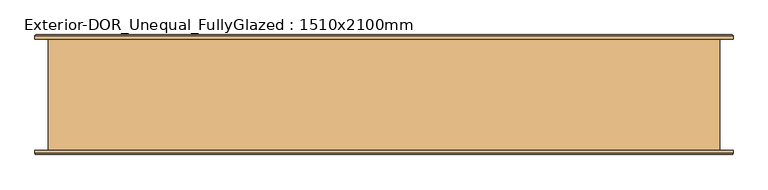
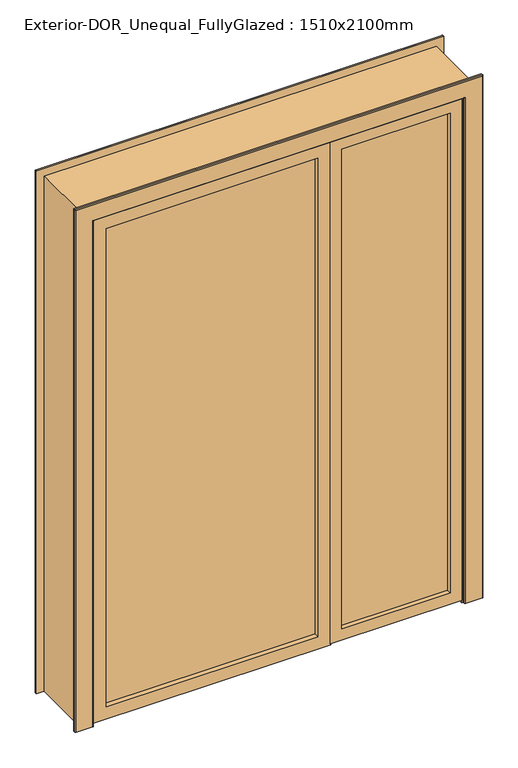
"""IFC4 building model written with IfcOpenShell, lengths in millimetres: door geometry, Exterior-DOR_Unequal_FullyGlazed : 1510x2100mm."""

import ifcopenshell
import ifcopenshell.guid

model = None  # the IFC model being written
_history = None  # IfcOwnerHistory: only IFC2X3 demands one
_inside = {}  # id of a spatial element -> (the spatial element, [elements in it])
_under = {}  # id of a project, library or spatial element -> (it, [spatial elements below it])
_declared = {}  # id of a project -> (the project, [libraries it declares])
_typed = {}  # id of a type object -> (the type object, [elements of that type])
_made_of = {}  # id of a material, layer set ... -> (it, [elements and type objects made of it])


def new_model(schema):
    """Start an empty IFC model of exactly this schema.

    Asked for "IFC4X3", IfcOpenShell would pick the latest addendum, in which some entities
    have other attributes; the version numbers below select the first issue.
    IFC2X3 requires an IfcOwnerHistory on every rooted entity: one is made here for all.
    """
    global model, _history
    if schema == "IFC4X3":
        model = ifcopenshell.file(schema_version=(4, 3, 0, 0))
    else:
        model = ifcopenshell.file(schema=schema)
    _inside.clear()
    _under.clear()
    _declared.clear()
    _typed.clear()
    _made_of.clear()
    _history = None
    if model.schema == "IFC2X3":
        org = make("IfcOrganization", Name="unknown")
        user = make(
            "IfcPersonAndOrganization",
            ThePerson=make("IfcPerson", FamilyName="unknown"),
            TheOrganization=org,
        )
        app = make(
            "IfcApplication",
            ApplicationDeveloper=org,
            Version="unknown",
            ApplicationFullName="unknown",
            ApplicationIdentifier="unknown",
        )
        _history = make(
            "IfcOwnerHistory",
            OwningUser=user,
            OwningApplication=app,
            ChangeAction="ADDED",
            CreationDate=0,
        )
    return model


def make(cls, **values):
    """One entity of the class cls with the attributes given. An attribute that is None is left unset."""
    return model.create_entity(
        cls, **{name: value for name, value in values.items() if value is not None}
    )


def rooted(cls, **values):
    """An entity with a GlobalId (a new one), such as an element, a storey or a relation."""
    return make(cls, GlobalId=ifcopenshell.guid.new(), OwnerHistory=_history, **values)


def si_unit(unit_type, name, prefix=None):
    """IfcSIUnit, for example si_unit("LENGTHUNIT", "METRE", prefix="MILLI")."""
    return make("IfcSIUnit", UnitType=unit_type, Prefix=prefix, Name=name)


def assignment(units):
    """IfcUnitAssignment: the units of a project."""
    return None if units is None else make("IfcUnitAssignment", Units=units)


def point(xyz):
    """IfcCartesianPoint."""
    return None if xyz is None else make("IfcCartesianPoint", Coordinates=xyz)


def direction(xyz):
    """IfcDirection."""
    return None if xyz is None else make("IfcDirection", DirectionRatios=xyz)


def frame(location, z_axis=None, x_axis=None):
    """IfcAxis2Placement3D, a coordinate frame: its origin and axes. An axis left out is left unset."""
    return make(
        "IfcAxis2Placement3D",
        Location=point(location),
        Axis=direction(z_axis),
        RefDirection=direction(x_axis),
    )


def origin():
    """The frame at (0, 0, 0) with its axes left unset."""
    return frame((0.0, 0.0, 0.0))


def place(relative_to, where):
    """IfcLocalPlacement: puts the frame where relative to a parent placement (None: the world)."""
    return make(
        "IfcLocalPlacement", PlacementRelTo=relative_to, RelativePlacement=where
    )


def context(
    kind, dimensions, precision=None, world=None, true_north=None, identifier=None
):
    """IfcGeometricRepresentationContext, for example the 3D "Model" context."""
    return make(
        "IfcGeometricRepresentationContext",
        ContextIdentifier=identifier,
        ContextType=kind,
        CoordinateSpaceDimension=dimensions,
        Precision=precision,
        WorldCoordinateSystem=world,
        TrueNorth=true_north,
    )


def project(units=None, contexts=None):
    """IfcProject with its units and contexts."""
    return rooted(
        "IfcProject",
        Name="project",
        RepresentationContexts=contexts,
        UnitsInContext=assignment(units),
    )


def spatial(cls, under=None, at=None, **own):
    """A site, building, storey or space (cls), placed at a placement, below another one or the project."""
    s = rooted(cls, ObjectPlacement=at, **own)
    if under is not None:
        _under.setdefault(under.id(), (under, []))[1].append(s)
    return s


def polyline(points):
    """IfcPolyline through the points."""
    return make("IfcPolyline", Points=[point(p) for p in points])


def circle_curve(where, radius):
    """IfcCircle in the frame where."""
    return make("IfcCircle", Position=where, Radius=radius)


def ellipse_curve(where, semi_axis1, semi_axis2):
    """IfcEllipse in the frame where."""
    return make(
        "IfcEllipse", Position=where, SemiAxis1=semi_axis1, SemiAxis2=semi_axis2
    )


def outline(outer, holes=None, kind="AREA"):
    """IfcArbitraryClosedProfileDef: a profile drawn as a closed curve; with holes, ...WithVoids."""
    if holes is None:
        return make("IfcArbitraryClosedProfileDef", ProfileType=kind, OuterCurve=outer)
    return make(
        "IfcArbitraryProfileDefWithVoids",
        ProfileType=kind,
        OuterCurve=outer,
        InnerCurves=holes,
    )


def extrude(swept, where, along, depth):
    """IfcExtrudedAreaSolid: the profile swept, set in the frame where, extruded along a direction by depth."""
    return make(
        "IfcExtrudedAreaSolid",
        SweptArea=swept,
        Position=where,
        ExtrudedDirection=direction(along),
        Depth=depth,
    )


def faces_of(points, faces, orient=None, outer=None):
    """IfcFace entities. A face is a list of loops; a loop is a list of indices into points, from 0.

    orient and outer hold one flag for each loop. By default every Orientation is true, the
    first loop of a face is its IfcFaceOuterBound and the others are IfcFaceBound.
    """
    made = []
    for i, loops in enumerate(faces):
        bounds = []
        for j, loop in enumerate(loops):
            is_outer = j == 0 if outer is None else outer[i][j]
            bounds.append(
                make(
                    "IfcFaceOuterBound" if is_outer else "IfcFaceBound",
                    Bound=make("IfcPolyLoop", Polygon=[points[k] for k in loop]),
                    Orientation=True if orient is None else orient[i][j],
                )
            )
        made.append(make("IfcFace", Bounds=bounds))
    return made


def faceted_brep(points, faces, orient=None, outer=None, voids=None):
    """IfcFacetedBrep: a solid bounded by flat faces; with voids (closed shells), ...WithVoids."""
    shared = [point(p) for p in points]
    hull = make("IfcClosedShell", CfsFaces=faces_of(shared, faces, orient, outer))
    if voids is None:
        return make("IfcFacetedBrep", Outer=hull)
    return make(
        "IfcFacetedBrepWithVoids",
        Outer=hull,
        Voids=[
            make(cls, CfsFaces=faces_of(shared, fs, o, b)) for cls, fs, o, b in voids
        ],
    )


def shape(context_of_items, identifier, shape_type, items):
    """IfcShapeRepresentation: the items that make up one representation, for example the "Body"."""
    return make(
        "IfcShapeRepresentation",
        ContextOfItems=context_of_items,
        RepresentationIdentifier=identifier,
        RepresentationType=shape_type,
        Items=items,
    )


def source(mapping_origin, context_of_items, identifier, shape_type, items):
    """IfcRepresentationMap: a shape defined once, which mapped items show again and again."""
    return make(
        "IfcRepresentationMap",
        MappingOrigin=mapping_origin,
        MappedRepresentation=shape(context_of_items, identifier, shape_type, items),
    )


def transform(
    local_origin,
    x_axis=None,
    y_axis=None,
    z_axis=None,
    scale=None,
    scale2=None,
    scale3=None,
    uniform=True,
):
    """IfcCartesianTransformationOperator3D, or its non-uniform kind. x_axis, y_axis, z_axis: its Axis1, 2, 3."""
    if uniform:
        return make(
            "IfcCartesianTransformationOperator3D",
            Axis1=direction(x_axis),
            Axis2=direction(y_axis),
            LocalOrigin=point(local_origin),
            Scale=scale,
            Axis3=direction(z_axis),
        )
    return make(
        "IfcCartesianTransformationOperator3DnonUniform",
        Axis1=direction(x_axis),
        Axis2=direction(y_axis),
        LocalOrigin=point(local_origin),
        Scale=scale,
        Axis3=direction(z_axis),
        Scale2=scale2,
        Scale3=scale3,
    )


def mapped(mapping_source, mapping_target):
    """IfcMappedItem: shows the shape of a source again, moved by a transform."""
    return make(
        "IfcMappedItem", MappingSource=mapping_source, MappingTarget=mapping_target
    )


def made_of(thing, what):
    """Note that an element or type object is made of a material, layer set ...; save() writes the relation."""
    if what is not None:
        _made_of.setdefault(what.id(), (what, []))[1].append(thing)
    return thing


def element(
    cls,
    number,
    at=None,
    inside=None,
    cuts=None,
    type_object=None,
    material=None,
    context=None,
    identifier="Body",
    shape_type=None,
    held_by="IfcProductDefinitionShape",
    body=None,
    shapes=None,
    **own,
):
    """One element of the class cls, such as IfcWall. Its Tag is "e" and its number.

    at: its placement. inside: the storey or other place that contains it. cuts: it is an
    opening in that element (IfcRelVoidsElement). A single representation is given by context,
    identifier, shape_type and body (its items); several are given by shapes. held_by: the class
    of the entity that holds the representations. save() writes the other relations.
    """
    e = rooted(cls, Tag="e%d" % number, ObjectPlacement=at, **own)
    if body is not None:
        shapes = [shape(context, identifier, shape_type, body)]
    if shapes is not None:
        e.Representation = make(held_by, Representations=shapes)
    if inside is not None:
        _inside.setdefault(inside.id(), (inside, []))[1].append(e)
    if cuts is not None:
        rooted(
            "IfcRelVoidsElement", RelatingBuildingElement=cuts, RelatedOpeningElement=e
        )
    if type_object is not None:
        _typed.setdefault(type_object.id(), (type_object, []))[1].append(e)
    return made_of(e, material)


def aggregate(whole, parts):
    """IfcRelAggregates: a whole, such as a stair, and the parts it consists of."""
    return rooted("IfcRelAggregates", RelatingObject=whole, RelatedObjects=parts)


def save(model, path):
    """Write the relations noted so far, then the file.

    IfcRelAggregates (storeys below a building ...), IfcRelContainedInSpatialStructure (elements
    in a storey), IfcRelDefinesByType, IfcRelAssociatesMaterial and IfcRelDeclares: one each for
    every whole, place, type object, material and project.
    """
    for whole, parts in _under.values():
        aggregate(whole, parts)
    for where, things in _inside.values():
        rooted(
            "IfcRelContainedInSpatialStructure",
            RelatedElements=things,
            RelatingStructure=where,
        )
    for kind, things in _typed.values():
        rooted("IfcRelDefinesByType", RelatedObjects=things, RelatingType=kind)
    for what, things in _made_of.values():
        rooted("IfcRelAssociatesMaterial", RelatedObjects=things, RelatingMaterial=what)
    for by, libraries in _declared.values():
        rooted("IfcRelDeclares", RelatingContext=by, RelatedDefinitions=libraries)
    model.write(path)


def plane_surface(at):
    """IfcPlane: the flat surface through the origin of the frame at, square to its z axis."""
    return make("IfcPlane", Position=at)


def cylinder_surface(at, radius):
    """IfcCylindricalSurface: all points at the distance radius from the z axis of the frame at."""
    return make("IfcCylindricalSurface", Position=at, Radius=radius)


def advanced_brep(points, edges, surfaces, faces):
    """IfcAdvancedBrep: a solid bounded by faces that lie on surfaces and meet in shared edges.

    An edge is (start, end): straight between two places in points (the first is 0);
    or (start, end, curve); or (start, end, curve, False) where it runs against its curve.
    A face is (place in surfaces, loops), or (place, loops, False) where it looks against
    its surface's normal. A loop lists edges by number (the first is 1), with a minus sign
    where the edge is run from its end to its start. The first loop is the outer one.
    """
    corners = [point(p) for p in points]
    vertices = [make("IfcVertexPoint", VertexGeometry=c) for c in corners]
    made = []
    for start, end, *more in edges:
        made.append(
            make(
                "IfcEdgeCurve",
                EdgeStart=vertices[start],
                EdgeEnd=vertices[end],
                EdgeGeometry=more[0] if more else make("IfcPolyline", Points=[corners[start], corners[end]]),
                SameSense=more[1] if len(more) > 1 else True,
            )
        )
    hull = []
    for where, loops, *sense in faces:
        bounds = []
        for j, loop in enumerate(loops):
            ring = [make("IfcOrientedEdge", EdgeElement=made[abs(k) - 1], Orientation=k > 0) for k in loop]
            bounds.append(
                make(
                    "IfcFaceOuterBound" if j == 0 else "IfcFaceBound",
                    Bound=make("IfcEdgeLoop", EdgeList=ring),
                    Orientation=True,
                )
            )
        hull.append(make("IfcAdvancedFace", Bounds=bounds, FaceSurface=surfaces[where], SameSense=sense[0] if sense else True))
    return make("IfcAdvancedBrep", Outer=make("IfcClosedShell", CfsFaces=hull))


def exterior_dor_unequal_fullyglazed_1510x2100mm_99816280(model_context):
    return source(origin(), model_context, "Body", "SolidModel", [
        extrude(outline(polyline([(247.5, -106.0), (247.5, -99.0), (665.0, -99.0), (665.0, -106.0), (247.5, -106.0)])), frame((0.0, 0.0, 55.0), z_axis=(0.0, 0.0, 1.0), x_axis=(1.0, 0.0, 0.0)), (0.0, 0.0, 1.0), 1955.0),
        extrude(outline(polyline([(10.0, 710.0), (2055.0, 710.0), (2055.0, 202.5), (10.0, 202.5), (10.0, 710.0)]), holes=[polyline([(2010.0, 247.5), (2010.0, 665.0), (55.0, 665.0), (55.0, 247.5), (2010.0, 247.5)])]), frame((0.0, -125.0, 0.0), z_axis=(0.0, 1.0, 0.0), x_axis=(0.0, 0.0, 1.0)), (0.0, 0.0, 1.0), 45.0),
        extrude(outline(polyline([(155.0, -106.0), (-660.0, -106.0), (-660.0, -99.0), (155.0, -99.0), (155.0, -106.0)])), frame((0.0, 0.0, 56.0), z_axis=(0.0, 0.0, 1.0), x_axis=(1.0, 0.0, 0.0)), (0.0, 0.0, 1.0), 1949.0),
        extrude(outline(polyline([(6.0, -710.0), (6.0, 205.0), (2055.0, 205.0), (2055.0, -710.0), (6.0, -710.0)]), holes=[polyline([(2005.0, 155.0), (56.0, 155.0), (56.0, -660.0), (2005.0, -660.0), (2005.0, 155.0)])]), frame((0.0, -125.0, 0.0), z_axis=(0.0, 1.0, 0.0), x_axis=(0.0, 0.0, 1.0)), (0.0, 0.0, 1.0), 45.0),
        advanced_brep(
        [(-715.0, -125.0, 0.0), (-715.0, -132.0, 0.0), (-718.0, -135.0, 0.0), (-782.0, -135.0, 0.0), (-785.0, -132.0, 0.0), (-785.0, -125.0, 0.0), (-715.0, -125.0, 2060.0), (-715.0, -132.0, 2060.0), (-718.0, -135.0, 2063.0), (718.0, -135.0, 2063.0), (718.0, -135.0, 0.0), (782.0, -135.0, 0.0), (782.0, -135.0, 2127.0), (-782.0, -135.0, 2127.0), (-785.0, -132.0, 2130.0), (-785.0, -125.0, 2130.0), (785.0, -125.0, 2130.0), (785.0, -125.0, 0.0), (715.0, -125.0, 0.0), (715.0, -125.0, 2060.0), (715.0, -132.0, 2060.0), (715.0, -132.0, 0.0), (785.0, -132.0, 0.0), (785.0, -132.0, 2130.0)],
        [
            (0, 1),
            (1, 2, circle_curve(frame((-718.0, -132.0, 0.0), z_axis=(0.0, 0.0, -1.0), x_axis=(-1.0, 0.0, 0.0)), 3.0)),
            (2, 3),
            (3, 4, circle_curve(frame((-782.0, -132.0, 0.0), z_axis=(0.0, 0.0, -1.0), x_axis=(-1.0, 0.0, 0.0)), 3.0)),
            (4, 5),
            (5, 0),
            (0, 6),
            (6, 7),
            (7, 1),
            (7, 8, ellipse_curve(frame((-718.0, -132.0, 2063.0), z_axis=(-0.7071067811865475, 0.0, -0.7071067811865475), x_axis=(0.7071067811865474, 0.0, -0.7071067811865476)), 4.2426407, 3.0)),
            (8, 2),
            (8, 9),
            (9, 10),
            (10, 11),
            (11, 12),
            (12, 13),
            (13, 3),
            (13, 14, ellipse_curve(frame((-782.0, -132.0, 2127.0), z_axis=(-0.7071067811865475, 0.0, -0.7071067811865475), x_axis=(0.7071067811865474, 0.0, -0.7071067811865476)), 4.2426407, 3.0)),
            (14, 4),
            (14, 15),
            (15, 5),
            (15, 16),
            (16, 17),
            (17, 18),
            (18, 19),
            (19, 6),
            (9, 20, ellipse_curve(frame((718.0, -132.0, 2063.0), z_axis=(0.7071067811865475, 0.0, -0.7071067811865475), x_axis=(0.7071067811865474, 0.0, 0.7071067811865476)), 4.2426407, 3.0)),
            (20, 21),
            (21, 10, circle_curve(frame((718.0, -132.0, 0.0), z_axis=(0.0, 0.0, 1.0), x_axis=(1.0, 0.0, 0.0)), 3.0)),
            (17, 22),
            (22, 11, circle_curve(frame((782.0, -132.0, 0.0), z_axis=(0.0, 0.0, -1.0), x_axis=(1.0, 0.0, 0.0)), 3.0)),
            (21, 18),
            (23, 12, ellipse_curve(frame((782.0, -132.0, 2127.0), z_axis=(0.7071067811865475, 0.0, -0.7071067811865475), x_axis=(0.7071067811865474, 0.0, 0.7071067811865476)), 4.2426407, 3.0)),
            (22, 23),
            (16, 23),
            (20, 19),
            (20, 7),
            (23, 14),
        ],
        [
            plane_surface(frame((-755.0, 125.0, 0.0), z_axis=(0.0, 0.0, -1.0), x_axis=(0.0, -1.0, 0.0))),
            plane_surface(frame((-715.0, -125.0, 0.0), z_axis=(1.0, 0.0, 0.0), x_axis=(0.0, 0.0, 1.0))),
            cylinder_surface(frame((-718.0, -132.0, 0.0), z_axis=(0.0, 0.0, -1.0), x_axis=(-1.0, 0.0, 0.0)), 3.0),
            plane_surface(frame((-718.0, -135.0, 0.0), z_axis=(0.0, -1.0, 0.0), x_axis=(0.0, 0.0, 1.0))),
            cylinder_surface(frame((-782.0, -132.0, 0.0), z_axis=(0.0, 0.0, -1.0), x_axis=(-1.0, 0.0, 0.0)), 3.0),
            plane_surface(frame((-785.0, -132.0, 0.0), z_axis=(-1.0, 0.0, 0.0), x_axis=(0.0, 0.0, 1.0))),
            plane_surface(frame((-785.0, -125.0, 0.0), z_axis=(0.0, 1.0, 0.0), x_axis=(0.0, 0.0, 1.0))),
            cylinder_surface(frame((718.0, -132.0, 2100.0), z_axis=(0.0, 0.0, 1.0), x_axis=(1.0, 0.0, 0.0)), 3.0),
            plane_surface(frame((755.0, 125.0, 0.0), z_axis=(0.0, 0.0, -1.0), x_axis=(0.0, -1.0, 0.0))),
            cylinder_surface(frame((782.0, -132.0, 2100.0), z_axis=(0.0, 0.0, 1.0), x_axis=(1.0, 0.0, 0.0)), 3.0),
            plane_surface(frame((785.0, -132.0, 2130.0), z_axis=(1.0, 0.0, 0.0), x_axis=(0.0, 0.0, -1.0))),
            plane_surface(frame((715.0, -125.0, 2060.0), z_axis=(-1.0, 0.0, 0.0), x_axis=(0.0, 0.0, -1.0))),
            plane_surface(frame((-715.0, -125.0, 2060.0), z_axis=(0.0, 0.0, -1.0), x_axis=(1.0, 0.0, 0.0))),
            cylinder_surface(frame((-755.0, -132.0, 2063.0), z_axis=(-1.0, 0.0, 0.0), x_axis=(0.0, 0.0, 1.0)), 3.0),
            cylinder_surface(frame((-755.0, -132.0, 2127.0), z_axis=(-1.0, 0.0, 0.0), x_axis=(0.0, 0.0, 1.0)), 3.0),
            plane_surface(frame((-785.0, -132.0, 2130.0), z_axis=(0.0, 0.0, 1.0), x_axis=(1.0, 0.0, 0.0))),
        ],
        [
            (0, [[1, 2, 3, 4, 5, 6]]),
            (1, [[-1, 7, 8, 9]]),
            (2, [[-2, -9, 10, 11]]),
            (3, [[-3, -11, 12, 13, 14, 15, 16, 17]]),
            (4, [[-4, -17, 18, 19]]),
            (5, [[-5, -19, 20, 21]]),
            (6, [[-6, -21, 22, 23, 24, 25, 26, -7]]),
            (7, [[27, 28, 29, -13]]),
            (8, [[-24, 30, 31, -14, -29, 32]]),
            (9, [[33, -15, -31, 34]]),
            (10, [[35, -34, -30, -23]]),
            (11, [[36, -25, -32, -28]]),
            (12, [[-8, -26, -36, 37]]),
            (13, [[-10, -37, -27, -12]]),
            (14, [[-18, -16, -33, 38]]),
            (15, [[-20, -38, -35, -22]]),
        ],
    ),
        advanced_brep(
        [(-785.0, 125.0, 0.0), (-785.0, 132.0, 0.0), (-782.0, 135.0, 0.0), (-718.0, 135.0, 0.0), (-715.0, 132.0, 0.0), (-715.0, 125.0, 0.0), (-785.0, 125.0, 2130.0), (-785.0, 132.0, 2130.0), (-782.0, 135.0, 2127.0), (782.0, 135.0, 2127.0), (782.0, 135.0, 0.0), (718.0, 135.0, 0.0), (718.0, 135.0, 2063.0), (-718.0, 135.0, 2063.0), (-715.0, 132.0, 2060.0), (-715.0, 125.0, 2060.0), (715.0, 125.0, 2060.0), (715.0, 125.0, 0.0), (785.0, 125.0, 0.0), (785.0, 125.0, 2130.0), (785.0, 132.0, 2130.0), (785.0, 132.0, 0.0), (715.0, 132.0, 0.0), (715.0, 132.0, 2060.0)],
        [
            (0, 1),
            (1, 2, circle_curve(frame((-782.0, 132.0, 0.0), z_axis=(0.0, 0.0, -1.0), x_axis=(-1.0, 0.0, 0.0)), 3.0)),
            (2, 3),
            (3, 4, circle_curve(frame((-718.0, 132.0, 0.0), z_axis=(0.0, 0.0, -1.0), x_axis=(-1.0, 0.0, 0.0)), 3.0)),
            (4, 5),
            (5, 0),
            (0, 6),
            (6, 7),
            (7, 1),
            (7, 8, ellipse_curve(frame((-782.0, 132.0, 2127.0), z_axis=(-0.7071067811865475, 0.0, -0.7071067811865475), x_axis=(0.7071067811865474, 0.0, -0.7071067811865476)), 4.2426407, 3.0)),
            (8, 2),
            (8, 9),
            (9, 10),
            (10, 11),
            (11, 12),
            (12, 13),
            (13, 3),
            (13, 14, ellipse_curve(frame((-718.0, 132.0, 2063.0), z_axis=(-0.7071067811865475, 0.0, -0.7071067811865475), x_axis=(0.7071067811865474, 0.0, -0.7071067811865476)), 4.2426407, 3.0)),
            (14, 4),
            (14, 15),
            (15, 5),
            (15, 16),
            (16, 17),
            (17, 18),
            (18, 19),
            (19, 6),
            (9, 20, ellipse_curve(frame((782.0, 132.0, 2127.0), z_axis=(0.7071067811865475, 0.0, -0.7071067811865475), x_axis=(0.7071067811865474, 0.0, 0.7071067811865476)), 4.2426407, 3.0)),
            (20, 21),
            (21, 10, circle_curve(frame((782.0, 132.0, 0.0), z_axis=(0.0, 0.0, 1.0), x_axis=(1.0, 0.0, 0.0)), 3.0)),
            (17, 22),
            (22, 11, circle_curve(frame((718.0, 132.0, 0.0), z_axis=(0.0, 0.0, -1.0), x_axis=(1.0, 0.0, 0.0)), 3.0)),
            (21, 18),
            (23, 12, ellipse_curve(frame((718.0, 132.0, 2063.0), z_axis=(0.7071067811865475, 0.0, -0.7071067811865475), x_axis=(0.7071067811865474, 0.0, 0.7071067811865476)), 4.2426407, 3.0)),
            (22, 23),
            (16, 23),
            (20, 19),
            (20, 7),
            (23, 14),
        ],
        [
            plane_surface(frame((-755.0, 125.0, 0.0), z_axis=(0.0, 0.0, -1.0), x_axis=(0.0, -1.0, 0.0))),
            plane_surface(frame((-785.0, 125.0, 0.0), z_axis=(-1.0, 0.0, 0.0), x_axis=(0.0, 0.0, 1.0))),
            cylinder_surface(frame((-782.0, 132.0, 0.0), z_axis=(0.0, 0.0, -1.0), x_axis=(-1.0, 0.0, 0.0)), 3.0),
            plane_surface(frame((-782.0, 135.0, 0.0), z_axis=(0.0, 1.0, 0.0), x_axis=(0.0, 0.0, 1.0))),
            cylinder_surface(frame((-718.0, 132.0, 0.0), z_axis=(0.0, 0.0, -1.0), x_axis=(-1.0, 0.0, 0.0)), 3.0),
            plane_surface(frame((-715.0, 132.0, 0.0), z_axis=(1.0, 0.0, 0.0), x_axis=(0.0, 0.0, 1.0))),
            plane_surface(frame((-715.0, 125.0, 0.0), z_axis=(0.0, -1.0, 0.0), x_axis=(0.0, 0.0, 1.0))),
            cylinder_surface(frame((782.0, 132.0, 2100.0), z_axis=(0.0, 0.0, 1.0), x_axis=(1.0, 0.0, 0.0)), 3.0),
            plane_surface(frame((755.0, 125.0, 0.0), z_axis=(0.0, 0.0, -1.0), x_axis=(0.0, -1.0, 0.0))),
            cylinder_surface(frame((718.0, 132.0, 2100.0), z_axis=(0.0, 0.0, 1.0), x_axis=(1.0, 0.0, 0.0)), 3.0),
            plane_surface(frame((715.0, 132.0, 2060.0), z_axis=(-1.0, 0.0, 0.0), x_axis=(0.0, 0.0, -1.0))),
            plane_surface(frame((785.0, 125.0, 2130.0), z_axis=(1.0, 0.0, 0.0), x_axis=(0.0, 0.0, -1.0))),
            plane_surface(frame((-785.0, 125.0, 2130.0), z_axis=(0.0, 0.0, 1.0), x_axis=(1.0, 0.0, 0.0))),
            cylinder_surface(frame((-755.0, 132.0, 2127.0), z_axis=(-1.0, 0.0, 0.0), x_axis=(0.0, 0.0, 1.0)), 3.0),
            cylinder_surface(frame((-755.0, 132.0, 2063.0), z_axis=(-1.0, 0.0, 0.0), x_axis=(0.0, 0.0, 1.0)), 3.0),
            plane_surface(frame((-715.0, 132.0, 2060.0), z_axis=(0.0, 0.0, -1.0), x_axis=(1.0, 0.0, 0.0))),
        ],
        [
            (0, [[1, 2, 3, 4, 5, 6]]),
            (1, [[-1, 7, 8, 9]]),
            (2, [[-2, -9, 10, 11]]),
            (3, [[-3, -11, 12, 13, 14, 15, 16, 17]]),
            (4, [[-4, -17, 18, 19]]),
            (5, [[-5, -19, 20, 21]]),
            (6, [[-6, -21, 22, 23, 24, 25, 26, -7]]),
            (7, [[27, 28, 29, -13]]),
            (8, [[-24, 30, 31, -14, -29, 32]]),
            (9, [[33, -15, -31, 34]]),
            (10, [[35, -34, -30, -23]]),
            (11, [[36, -25, -32, -28]]),
            (12, [[-8, -26, -36, 37]]),
            (13, [[-10, -37, -27, -12]]),
            (14, [[-18, -16, -33, 38]]),
            (15, [[-20, -38, -35, -22]]),
        ],
    ),
        faceted_brep([(-755.0, 125.0, 0.0), (-710.0, 125.0, 0.0), (-710.0, -40.0, 0.0), (-690.0, -40.0, 0.0), (-690.0, -80.0, 0.0), (-710.0, -80.0, 0.0), (-710.0, -125.0, 0.0), (-755.0, -125.0, 0.0), (-755.0, 125.0, 2100.0), (755.0, 125.0, 2100.0), (755.0, 125.0, 0.0), (710.0, 125.0, 0.0), (710.0, 125.0, 2055.0), (-710.0, 125.0, 2055.0), (-710.0, -40.0, 2055.0), (710.0, -40.0, 2055.0), (710.0, -40.0, 0.0), (690.0, -40.0, 0.0), (690.0, -40.0, 2035.0), (-690.0, -40.0, 2035.0), (-690.0, -80.0, 2035.0), (690.0, -80.0, 2035.0), (690.0, -80.0, 0.0), (710.0, -80.0, 0.0), (710.0, -80.0, 2055.0), (-710.0, -80.0, 2055.0), (-710.0, -125.0, 2055.0), (710.0, -125.0, 2055.0), (710.0, -125.0, 0.0), (755.0, -125.0, 0.0), (755.0, -125.0, 2100.0), (-755.0, -125.0, 2100.0)], [[[0, 1, 2, 3, 4, 5, 6, 7]], [[1, 0, 8, 9, 10, 11, 12, 13]], [[2, 1, 13, 14]], [[3, 2, 14, 15, 16, 17, 18, 19]], [[4, 3, 19, 20]], [[5, 4, 20, 21, 22, 23, 24, 25]], [[6, 5, 25, 26]], [[7, 6, 26, 27, 28, 29, 30, 31]], [[0, 7, 31, 8]], [[9, 30, 29, 10]], [[10, 29, 28, 23, 22, 17, 16, 11]], [[15, 12, 11, 16]], [[21, 18, 17, 22]], [[27, 24, 23, 28]], [[20, 19, 18, 21]], [[26, 25, 24, 27]], [[8, 31, 30, 9]], [[14, 13, 12, 15]]]),
    ])


if __name__ == "__main__":
    model = new_model("IFC4")
    model_context = context("Model", 3, world=origin())
    ifc_project = project(units=[si_unit("LENGTHUNIT", "METRE", prefix="MILLI")], contexts=[model_context])
    site = spatial("IfcSite", under=ifc_project)
    building = spatial("IfcBuilding", under=site)
    placement = place(None, origin())
    exterior_dor_unequal_fullyglazed_1510x2100mm_shape = exterior_dor_unequal_fullyglazed_1510x2100mm_99816280(model_context)
    element("IfcDoor", 1, ObjectType="Exterior-DOR_Unequal_FullyGlazed : 1510x2100mm", at=placement, inside=building, context=model_context, shape_type="MappedRepresentation", body=[
        mapped(exterior_dor_unequal_fullyglazed_1510x2100mm_shape, transform((0.0, 0.0, 0.0), x_axis=(1.0, 0.0, 0.0), y_axis=(0.0, 1.0, 0.0), z_axis=(0.0, 0.0, 1.0))),
    ])
    save(model, "model.ifc")

# Revit data of these elements
# Type "Exterior-DOR_Unequal_FullyGlazed : 1510x2100mm"
#   Type IfcGUID = "2NKTNbJKP36hSTtB23uCk3"
#   Assembly Code = "B2030100"
#   Type Mark = "190"
#   Classification.Uniclass.EF.Number = "EF_25_30"
#   Classification.Uniclass.EF.Description = "Doors and windows"
#   WindLoadRating = "n/a"
#   WaterTightnessRating = "n/a"
#   WarrantyStartDate [instance default] = "1900-12-31T23:59:59"
#   WarrantyGuarantorParts = "n/a"
#   WarrantyGuarantorLabor = "n/a"
#   WarrantyDurationUnit = "year"
#   WarrantyDurationParts = "n/a"
#   WarrantyDurationLabor = "n/a"
#   WarrantyDescription = "n/a"
#   Version = "2"
#   Uniclass2015Version = "Systems v1.9"
#   Uniclass2015Title = "Doorset systems"
#   Uniclass2015Code = "Ss_25_30_20_25"
#   URL = "www.nationalbimlibrary.com"
#   TagNumber [instance default] = "n/a"
#   SustainabilityPerformance = "n/a"
#   Status = "UNSET"
#   Size = "1510 x 2100 mm"
#   Shape = "n/a"
#   SerialNumber [instance default] = "n/a"
#   SecurityRating = "n/a"
#   Revision = "n/a"
#   ReplacementCost = "n/a"
#   Reference = "n/a"
#   ProductInformation = "n/a"
#   Operation = "DOUBLE_DOOR_SINGLE_SWING"
#   OmniClassVersion = "Table 22 2012-05-16"
#   OmniClassTitle = "Doors and Frames"
#   OmniClassCode = "22-08 10 00"
#   Name = "DoorsetSystem_Interior-Unequal_FullGlazed"
#   NBSReference = "25-50-20/120"
#   NBSDescription = "Doorset system"
#   NBSCertification = "www.nationalbimlibrary.com/cert/fxtqd0eu"
#   ModelReference = "Interior Unequal Door Fully Glazed Leaf"
#   ModelNumber = "n/a"
#   Model = "Interior Unequal Door Fully Glazed Leaf"
#   MechanicalLoadRating = "n/a"
#   Material = "n/a"
#   ManufacturerURL = "n/a"
#   ManufacturerName = "n/a"
#   Manufacturer = "info@theNBS.com"
#   InstallationDate [instance default] = "1900-12-31T23:59:59"
#   IfcExportType = "DOOR"
#   IfcExportAs = "IfcDoorType"
#   HygrothermalRating = "n/a"
#   Grade = "n/a"
#   GlassColor = "n/a"
#   FireRating = "n/a"
#   Fire Rating = "n/a"
#   Finish = "n/a"
#   FillGas = "n/a"
#   Features = "n/a"
#   ExpectedLife = "n/a"
#   DurationUnit = "n/a"
#   DurabilityRating = "n/a"
#   DoorNumber [instance default] = "n/a"
#   Description = "Generic unequal interior door with fully glazed leaf"
#   Construction Type = "ALUMINIUM"
#   Constituents = "n/a"
#   ComponentNumber [instance default] = "n/a"
#   Color = "n/a"
#   CodePerformance = "n/a"
#   Category = "Ss_25_30_20_25:Doorset systems"
#   BarCode [instance default] = "n/a"
#   BIMObjectName = "NBS_DoorsetSystem_Interior-Unequal_FullyGlazed"
#   Author = "NBS"
#   AssetType = "Fixed"
#   AssetIdentifier [instance default] = "n/a"
#   Analytic Construction = "<None>"
#   AcousticRating = "n/a"
#   AccessibilityPerformance = "n/a"
#   Width = 1.51 m
#   WallThickness [instance default] = 0.15 m
#   VisibleLightTransmittance = 0
#   VisibileLightReflectance = 0
#   Thickness = 0.15 m
#   ThermalTransmittanceWinter = 0
#   ThermalTransmittanceSummer = 0
#   ThermalTransmittance = 0
#   StructuralToleranceJamb = 0 m
#   StructuralToleranceHead = 0 m
#   StructuralOpeningWidth = 1.51 m
#   StructuralOpeningHeight = 2.1 m
#   StopProjection = 0.02 m
#   StopDepth = 0.04 m
#   SolarTransmittance = 0
#   SolarReflectance = 0
#   SolarHeatGainTransmittance = 0
#   SolarAbsorption = 0
#   ShadingCoefficient = 0
#   SecondaryPanelWidth = 0.5075 m
#   Rough Width [instance default] = 1.51 m
#   Rough Height [instance default] = 2.1 m
#   RebateDepth = 0.045 m
#   PanelUndercut = 0.006 m
#   PanelHeight = 2.055 m
#   PanelDepth = 0.045 m
#   OpeningTolerance = 0 m
#   NominalWidth = 1.51 m
#   NominalLength = 0 m
#   NominalHeight = 2.1 m
#   MeetingStileTolerance = 0.0025 m
#   MainPanelWidth = 0.91 m
#   Infiltration = 0
#   Height = 2.1 m
#   GlazingPanelWidth = 0.2 m
#   GlazingPanelThickness = 0.007 m
#   GlazingPanelDiameter = 0.4 m
#   GlazingPanelCentre = 1.6 m
#   GlazingOffsetFromEdgeOfPanel = 0.2 m
#   GlazingOffsetFromBottomOfPanel = 1.106 m
#   GlazingAreaFraction = 0
#   GlassThickness3 = 0.002 m
#   GlassThickness2 = 0.002 m
#   GlassThickness1 = 0.002 m
#   FrameThickness = 0.045 m
#   FrameSetback [instance default] = 0 m
#   FrameDepth [instance default] = 0.15 m
#   FinishThicknessInternal [instance default] = 0 m
#   FinishThicknessExternal [instance default] = 0 m
#   ClearOpeningWidth = 1.38 m
#   ClearOpeningHeight = 2.035 m
#   CalculatedInteriorVoidDepth [instance default] = 0.3 m
#   ArchitraveWidth = 0.07 m
#   ArchitraveThickness = 0.01 m
#   ArchitraveSetbackFromFrameFace = 0.005 m
#   SmokeStop = no
#   SingleRebate = no
#   SelfClosing = no
#   PlantedStop = yes
#   IsWired = no
#   IsTempered = no
#   IsLaminated = no
#   IsExternal = yes
#   IsCoated = no
#   HasDrive = no
#   HandicapAccessible = no
#   GlassLayers = 3
#   Function = 1
#   Wall Closure = 4
#   FireExit = no
#   ArchitraveFrontRequired [instance default] = yes
#   ArchitraveBackRequired [instance default] = yes
#   PanelMaterial = NBS_Concept
#   GlazingPanelMaterial = NBS_Glass_Single
#   GlazingBeadMaterial = NBS_Concept
#   FrameSectionMaterial = NBS_Concept
#   Cost = 0
# Element 1 (IfcDoor, "Exterior-DOR_Unequal_FullyGlazed : 1510x2100mm")
#   WallThickness = 0.25 m
#   FrameDepth = 0.25 m
#   Materials on its faces: "NBS_Concept", "NBS_Glass_Single"
# Materials
#   "NBS_Concept": class "Generic", colour RGB 255 255 255, transparency 0, Description = "To be specified", Cost = 0
#   "NBS_Glass_Single": class "Glass", colour RGB 94 140 251, transparency 0.6, Cost = 0
